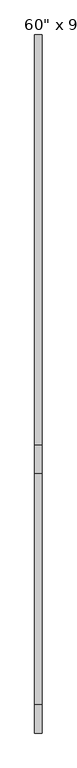
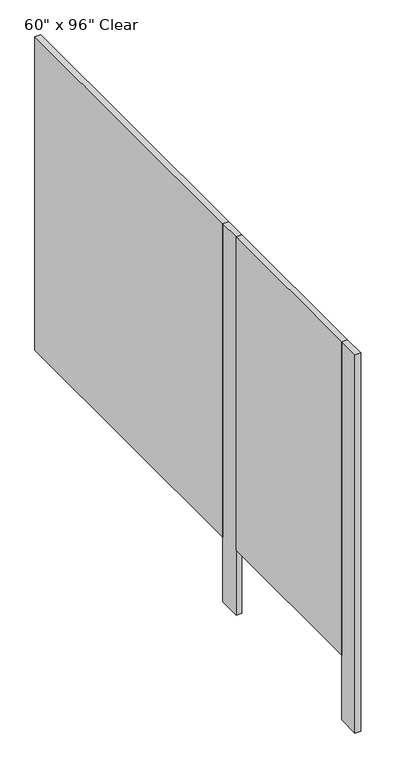
"""IFC4 building model written with IfcOpenShell, lengths in millimetres: proxy geometry."""

from ifc_helpers import new_model, si_unit, frame, origin, origin_with_axes, place, context, project, spatial, polyline, outline, extrude, source, transform, mapped, element, save


def proxy_f18b863e(model_context):
    return source(origin(), model_context, "Body", "SweptSolid", [
        extrude(outline(polyline([(-661.8968462, -2560.6375), (-687.2968462, -2560.6375), (-687.2968462, -1747.8375), (-661.8968462, -1747.8375), (-661.8968462, -2560.6375)])), frame((0.0, 0.0, 304.8), z_axis=(0.0, 0.0, 1.0), x_axis=(1.0, 0.0, 0.0)), (0.0, 0.0, 1.0), 1473.2),
        extrude(outline(polyline([(-661.8968462, -2662.2375), (-687.2968462, -2662.2375), (-687.2968462, -2560.6375), (-661.8968462, -2560.6375), (-661.8968462, -2662.2375)])), origin_with_axes(), (0.0, 0.0, 1.0), 1778.0),
        extrude(outline(polyline([(-661.8968462, -1747.8375), (-687.2968462, -1747.8375), (-687.2968462, -1646.2375), (-661.8968462, -1646.2375), (-661.8968462, -1747.8375)])), origin_with_axes(), (0.0, 0.0, 1.0), 1778.0),
        extrude(outline(polyline([(-687.2968462, -1646.2375), (-687.2968462, -198.4375), (-661.8968462, -198.4375), (-661.8968462, -1646.2375), (-687.2968462, -1646.2375)])), frame((0.0, 0.0, 304.8), z_axis=(0.0, 0.0, 1.0), x_axis=(1.0, 0.0, 0.0)), (0.0, 0.0, 1.0), 1473.2),
    ])


if __name__ == "__main__":
    model = new_model("IFC4")
    model_context = context("Model", 3, world=origin())
    ifc_project = project(units=[si_unit("LENGTHUNIT", "METRE", prefix="MILLI")], contexts=[model_context])
    site = spatial("IfcSite", under=ifc_project)
    building = spatial("IfcBuilding", under=site)
    placement = place(None, origin())
    proxy_shape = proxy_f18b863e(model_context)
    element("IfcBuildingElementProxy", 1, Name="Toilet Stall-Accessible-Side-3D w Toilet : 60\" x 96\" Clear", ObjectType="Toilet Stall-Accessible-Side-3D w Toilet : 60\" x 96\" Clear", at=placement, inside=building, context=model_context, shape_type="MappedRepresentation", body=[
        mapped(proxy_shape, transform((0.0, 0.0, 0.0), x_axis=(1.0, 0.0, 0.0), y_axis=(0.0, 1.0, 0.0), z_axis=(0.0, 0.0, 1.0))),
    ])
    save(model, "model.ifc")

# Revit data of these elements
# Type "Toilet Stall-Accessible-Side-3D w Toilet : 60\" x 96\" Clear"
#   Assembly Code = "C1030100"
#   Door Width = 2' - 8"
#   Length = 8' - 0"
#   Width = 5' - 0"
#   Show End Panel [instance default] = yes
#   Toilet Partition Material = Toilet Partition
#   Default Elevation = 0
# Element 1 (IfcBuildingElementProxy, "Toilet Stall-Accessible-Side-3D w Toilet : 60\" x 96\" Clear")
#   Show End Panel = no
#   Materials on its faces: "Toilet Partition"
# Materials
#   "Toilet Partition": class "Unassigned", colour RGB 0 181 188, transparency 0
